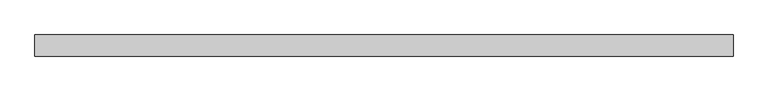
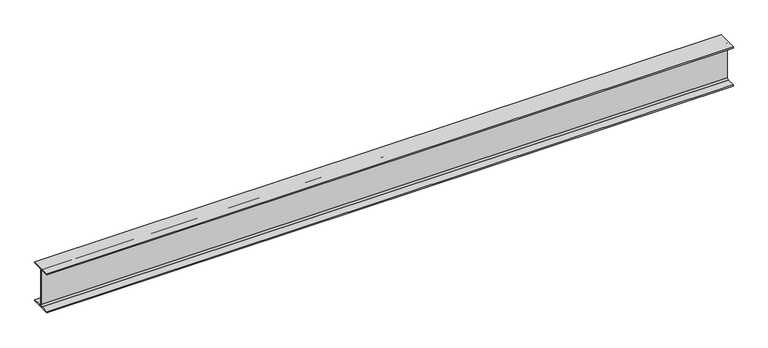
"""IFC4 building model written with IfcOpenShell, lengths in millimetres: beam geometry, 0912_Steel Framing_H-KSD3502 : H_SB_ASB_H-350x175x7x11."""

from ifc_helpers import new_model, si_unit, point, frame, frame_2d, origin, place, context, project, spatial, polyline, circle_curve, trimmed, segment, composite_curve, outline, extrude, source, transform, mapped, element, save


def beam_53bde3f6(model_context):
    return source(origin(), model_context, "Body", "SweptSolid", [
        extrude(outline(composite_curve([segment(polyline([(87.5, -164.0), (87.5, -175.0), (-87.5, -175.0), (-87.5, -164.0), (-17.5, -164.0)]), True, "CONTINUOUS"), segment(trimmed(circle_curve(frame_2d((-17.5, -150.0)), 14.0), [point((-17.5, -164.0))], [point((-3.5, -150.0))], True, "CARTESIAN"), True, "CONTINUOUS"), segment(polyline([(-3.5, -150.0), (-3.5, 150.0)]), True, "CONTINUOUS"), segment(trimmed(circle_curve(frame_2d((-17.5, 150.0)), 14.0), [point((-3.5, 150.0))], [point((-17.5, 164.0))], True, "CARTESIAN"), True, "CONTINUOUS"), segment(polyline([(-17.5, 164.0), (-87.5, 164.0), (-87.5, 175.0), (87.5, 175.0), (87.5, 164.0), (17.5, 164.0)]), True, "CONTINUOUS"), segment(trimmed(circle_curve(frame_2d((17.5, 150.0)), 14.0), [point((17.5, 164.0))], [point((3.5, 150.0))], True, "CARTESIAN"), True, "CONTINUOUS"), segment(polyline([(3.5, 150.0), (3.5, -150.0)]), True, "CONTINUOUS"), segment(trimmed(circle_curve(frame_2d((17.5, -150.0)), 14.0), [point((3.5, -150.0))], [point((17.5, -164.0))], True, "CARTESIAN"), True, "CONTINUOUS"), segment(polyline([(17.5, -164.0), (87.5, -164.0)]), True, "CONTINUOUS")], self_intersect=False)), frame((-2769.2350039, 0.0, 0.0), z_axis=(1.0, 0.0, 0.0), x_axis=(0.0, 1.0, 0.0)), (0.0, 0.0, 1.0), 5784.1976903),
    ])


if __name__ == "__main__":
    model = new_model("IFC4")
    model_context = context("Model", 3, world=origin())
    ifc_project = project(units=[si_unit("LENGTHUNIT", "METRE", prefix="MILLI")], contexts=[model_context])
    site = spatial("IfcSite", under=ifc_project)
    building = spatial("IfcBuilding", under=site)
    placement = place(None, origin())
    beam_shape = beam_53bde3f6(model_context)
    element("IfcBeam", 1, ObjectType="0912_Steel Framing_H-KSD3502 : H_SB_ASB_H-350x175x7x11", at=placement, inside=building, context=model_context, shape_type="MappedRepresentation", body=[
        mapped(beam_shape, transform((0.0, 0.0, 0.0), x_axis=(1.0, 0.0, 0.0), y_axis=(0.0, 1.0, 0.0), z_axis=(0.0, 0.0, 1.0))),
    ])
    save(model, "model.ifc")

# Revit data of these elements
# Type "0912_Steel Framing_H-KSD3502 : H_SB_ASB_H-350x175x7x11"
#   H_WM Code_1 = "S01AA002-00001 | Main Steel Structure Fabrication Work | Shelter/Building | Medium Steel - Standard (90KG/M>Weight≥30KG/M) | Material: (   )"
#   H_WM Code_2 = "S03AA028-00001 | Main Steel Structure Erection Work | Shelter/Building | Medium Steel (90KG/M>Weight≥30KG/M) | Material: (   )"
#   H_WM Code_3 = "S01AA010-00001 | Main Steel Structure Fabrication Work | Shelter/Building | Steel Painting/Coating | for Non-Fireproofed Steel Surface, Surface Preparation, Primer, Second & Final Coat | Material: (   )"
#   H_Q'ty Cal Type Tag = "SB-Q2"
#   Width = 17.5 cm
#   Web Thickness = 0.7 cm
#   Web Fillet = 1.4 cm
#   Warping Constant = 282000.0 cm⁶
#   W = 0
#   Torsional Moment of Inertia = 19.4042 cm⁴
#   Section Area = 63.14 cm²
#   Plastic Modulus weak axis = 174.0 cm³
#   Plastic Modulus strong axis = 868.0 cm³
#   Perimeter = 1.36 m²/m
#   Nominal Weight = 49.60 kgf/m
#   Moment of Inertia weak axis = 984.00 cm⁴
#   Moment of Inertia strong axis = 13600.00 cm⁴
#   Height = 35.0 cm
#   Flange Thickness = 1.1 cm
#   Elastic Modulus weak axis = 112.0 cm³
#   Elastic Modulus strong axis = 775.0 cm³
#   Centroid Vertical = 17.5 cm
#   Centroid Horizontal = 8.75 cm
#   Ix = 136000000
#   Length [instance default] = 1.5240 m
#   Zx = 868000
#   b = 0.1750 m
#   h = 0.3500 m
#   r = 0.0140 m
#   s = 0.0070 m
#   t = 0.0110 m
#   A = 0.006314 m²
#   Structural Material [instance default] = Steel, 45-345
#   Assembly Code = ""
# Element 1 (IfcBeam, "0912_Steel Framing_H-KSD3502 : H_SB_ASB_H-350x175x7x11")
#   Structural Material = none
# Materials
#   "Steel, 45-345": class "Metal", colour RGB 189 187 185, transparency 0, Description = "Steel 345 MPa", Cost = 0
